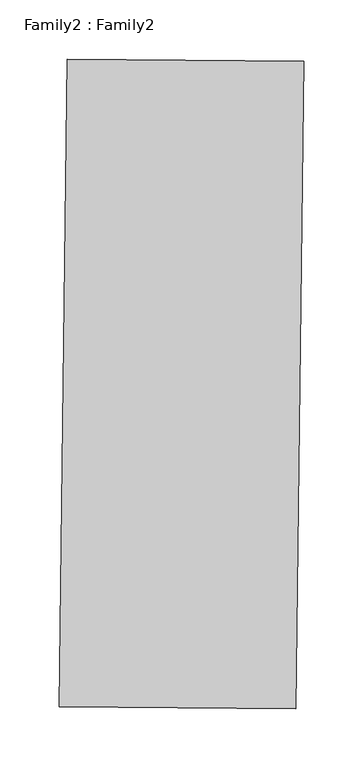
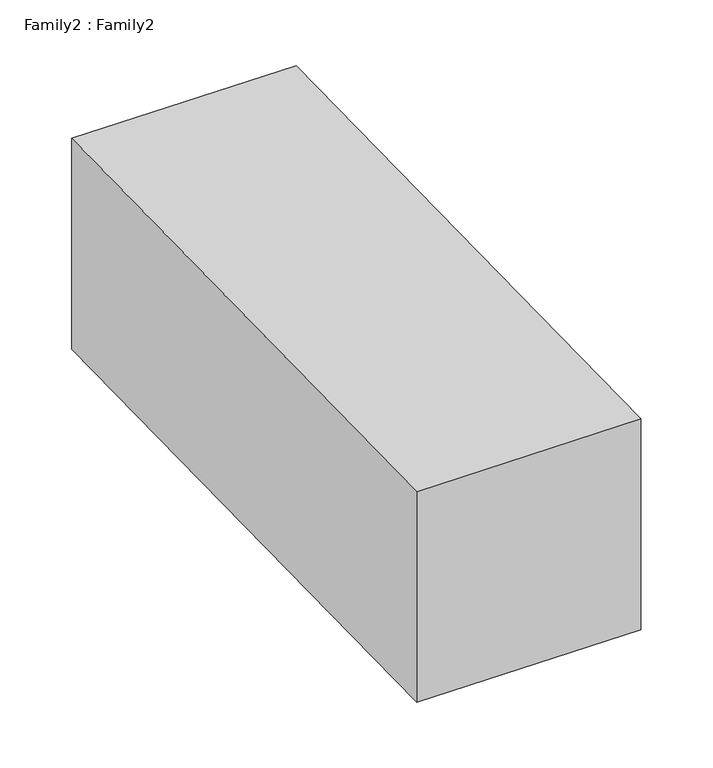
"""IFC4 building model written with IfcOpenShell, lengths in millimetres: proxy geometry, Family2 : Family2."""

from ifc_helpers import new_model, si_unit, origin, place, context, project, spatial, faceted_brep, source, transform, mapped, element, save


def family2_family2_2f13623d(model_context):
    return source(origin(), model_context, "Body", "Brep", [
        faceted_brep([(-3946.8046564, -6347.4583376, 1.0945136), (-3946.8046564, -6347.4583376, 201.0945136), (-3940.0381381, -5800.141785, 202.060409), (-3940.0381381, -5800.141785, 2.060409), (-3746.8134664, -6349.3355503, 201.0945136), (-3740.0469481, -5802.0189977, 202.060409), (-3746.8134664, -6349.3355503, 1.0945136), (-3740.0469481, -5802.0189977, 2.060409)], [[[0, 1, 2, 3]], [[1, 4, 5, 2]], [[4, 6, 7, 5]], [[6, 0, 3, 7]], [[3, 2, 5, 7]], [[0, 6, 4, 1]]]),
    ])


if __name__ == "__main__":
    model = new_model("IFC4")
    model_context = context("Model", 3, world=origin())
    ifc_project = project(units=[si_unit("LENGTHUNIT", "METRE", prefix="MILLI")], contexts=[model_context])
    site = spatial("IfcSite", under=ifc_project)
    building = spatial("IfcBuilding", under=site)
    placement = place(None, origin())
    family2_family2_shape = family2_family2_2f13623d(model_context)
    element("IfcBuildingElementProxy", 1, Name="Family2 : Family2", ObjectType="Family2 : Family2", at=placement, inside=building, context=model_context, shape_type="MappedRepresentation", body=[
        mapped(family2_family2_shape, transform((0.0, 0.0, 0.0), x_axis=(1.0, 0.0, 0.0), y_axis=(0.0, 1.0, 0.0), z_axis=(0.0, 0.0, 1.0))),
    ])
    save(model, "model.ifc")

# Revit data of these elements
# Type "Family2 : Family2"
#   Default Elevation = 0
